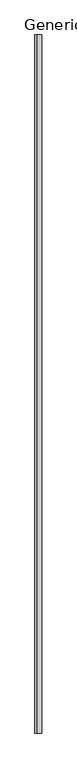
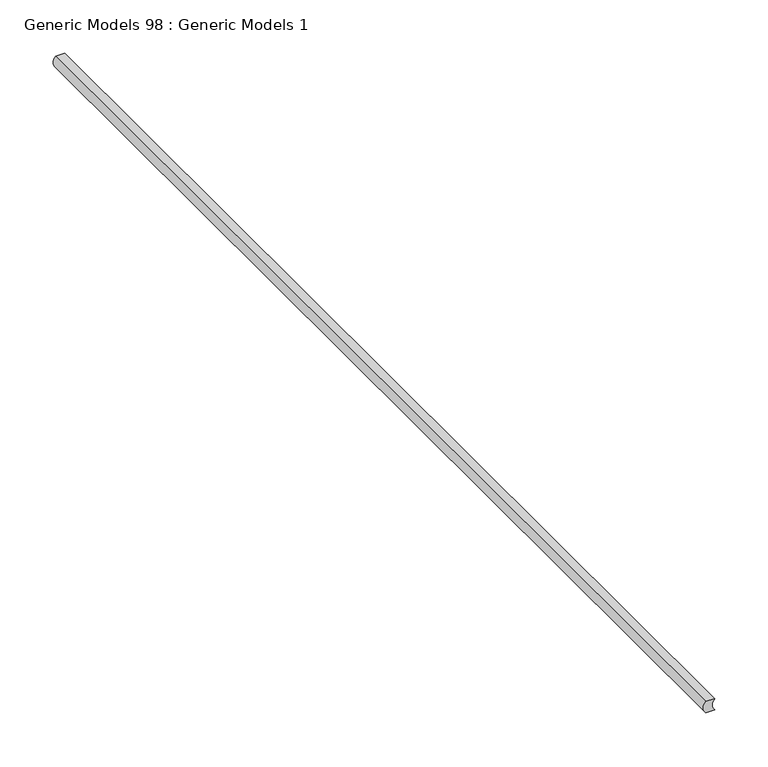
"""IFC4 building model written with IfcOpenShell, lengths in millimetres: proxy geometry, Generic Models 98 : Generic Models 1."""

from ifc_helpers import new_model, si_unit, point, frame, frame_2d, origin, place, context, project, spatial, polyline, circle_curve, trimmed, segment, composite_curve, outline, extrude, source, transform, mapped, element, save


def generic_models_98_generic_models_1_309ea474(model_context):
    return source(origin(), model_context, "Body", "SweptSolid", [
        extrude(outline(composite_curve([segment(trimmed(circle_curve(frame_2d((2225.123933, 46957.578034)), 8.620055), [point((2218.773933, 46951.7485531))], [point((2231.473933, 46951.7485531))], True, "CARTESIAN"), True, "CONTINUOUS"), segment(polyline([(2231.473933, 46951.7485531), (2231.473933, 46942.2235531)]), True, "CONTINUOUS"), segment(trimmed(circle_curve(frame_2d((2225.123933, 46948.053034)), 8.620055), [point((2231.473933, 46942.2235531))], [point((2218.773933, 46942.2235531))], False, "CARTESIAN"), True, "CONTINUOUS"), segment(polyline([(2218.773933, 46942.2235531), (2218.773933, 46951.7485531)]), True, "CONTINUOUS")], self_intersect=False)), frame((0.0, 0.0, 0.0), z_axis=(0.0, 1.0, 0.0), x_axis=(0.0, 0.0, 1.0)), (0.0, 0.0, 1.0), 1219.2),
    ])


if __name__ == "__main__":
    model = new_model("IFC4")
    model_context = context("Model", 3, world=origin())
    ifc_project = project(units=[si_unit("LENGTHUNIT", "METRE", prefix="MILLI")], contexts=[model_context])
    site = spatial("IfcSite", under=ifc_project)
    building = spatial("IfcBuilding", under=site)
    placement = place(None, origin())
    generic_models_98_generic_models_1_shape = generic_models_98_generic_models_1_309ea474(model_context)
    element("IfcBuildingElementProxy", 1, Name="Generic Models 98 : Generic Models 1", ObjectType="Generic Models 98 : Generic Models 1", at=placement, inside=building, context=model_context, shape_type="MappedRepresentation", body=[
        mapped(generic_models_98_generic_models_1_shape, transform((0.0, 0.0, 0.0), x_axis=(1.0, 0.0, 0.0), y_axis=(0.0, 1.0, 0.0), z_axis=(0.0, 0.0, 1.0))),
    ])
    save(model, "model.ifc")

# Revit data of these elements
# Element 1 (IfcBuildingElementProxy, "Generic Models 98 : Generic Models 1")
#   Materials on its faces: "SEALANT (W/ BACKER ROD IF NECESSARY)"
# Materials
#   "SEALANT (W/ BACKER ROD IF NECESSARY)": class "Unassigned", colour RGB 120 120 120, transparency 0, Cost = 0
